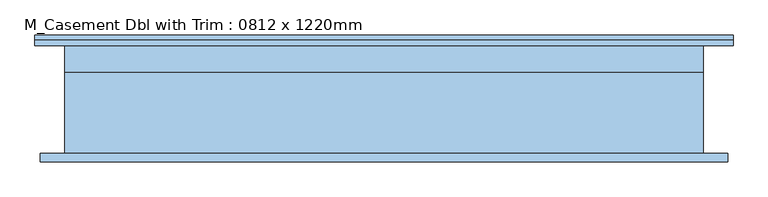
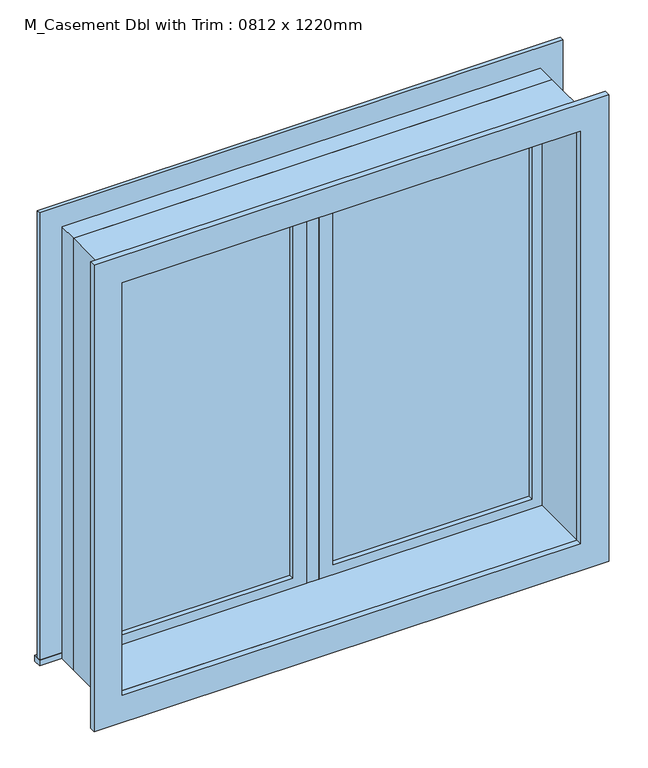
"""IFC4 building model written with IfcOpenShell, lengths in millimetres: window geometry, M_Casement Dbl with Trim : 0812 x 1220mm."""

from ifc_helpers import new_model, si_unit, frame, origin, place, context, project, spatial, polyline, outline, extrude, source, transform, mapped, element, save


def m_casement_dbl_with_trim_0812_x_1220mm_81b237b5(model_context):
    return source(origin(), model_context, "Body", "SweptSolid", [
        extrude(outline(polyline([(63.5, 111.175), (686.5, 111.175), (686.5, 98.475), (63.5, 98.475), (63.5, 111.175)])), frame((0.0, 0.0, 963.5), z_axis=(0.0, 0.0, 1.0), x_axis=(1.0, 0.0, 0.0)), (0.0, 0.0, 1.0), 1303.0),
        extrude(outline(polyline([(2310.95, 19.05), (919.05, 19.05), (919.05, 730.95), (2310.95, 730.95), (2310.95, 19.05)]), holes=[polyline([(2266.5, 63.5), (2266.5, 686.5), (963.5, 686.5), (963.5, 63.5), (2266.5, 63.5)])]), frame((0.0, 82.6, 0.0), z_axis=(0.0, 1.0, 0.0), x_axis=(0.0, 0.0, 1.0)), (0.0, 0.0, 1.0), 44.45),
        extrude(outline(polyline([(-819.95, 171.75), (819.95, 171.75), (819.95, 146.05), (-819.95, 146.05), (-819.95, 171.75)])), frame((0.0, 0.0, 900.0), z_axis=(0.0, 0.0, 1.0), x_axis=(1.0, 0.0, 0.0)), (0.0, 0.0, 1.0), 19.05),
        extrude(outline(polyline([(2310.95, -730.95), (2310.95, 730.95), (919.05, 730.95), (919.05, 819.95), (2399.95, 819.95), (2399.95, -819.95), (919.05, -819.95), (919.05, -730.95), (2310.95, -730.95)])), frame((0.0, 146.05, 0.0), z_axis=(0.0, 1.0, 0.0), x_axis=(0.0, 0.0, 1.0)), (0.0, 0.0, 1.0), 13.0),
        extrude(outline(polyline([(2387.25, 807.25), (2387.25, -807.25), (842.75, -807.25), (842.75, 807.25), (2387.25, 807.25)]), holes=[polyline([(2298.25, 718.25), (931.75, 718.25), (931.75, -718.25), (2298.25, -718.25), (2298.25, 718.25)])]), frame((0.0, -126.95, 0.0), z_axis=(0.0, 1.0, 0.0), x_axis=(0.0, 0.0, 1.0)), (0.0, 0.0, 1.0), 19.0),
        extrude(outline(polyline([(-63.5, 98.475), (-686.5, 98.475), (-686.5, 111.175), (-63.5, 111.175), (-63.5, 98.475)])), frame((0.0, 0.0, 963.5), z_axis=(0.0, 0.0, 1.0), x_axis=(1.0, 0.0, 0.0)), (0.0, 0.0, 1.0), 1303.0),
        extrude(outline(polyline([(2310.95, -730.95), (919.05, -730.95), (919.05, -19.05), (2310.95, -19.05), (2310.95, -730.95)]), holes=[polyline([(2266.5, -686.5), (2266.5, -63.5), (963.5, -63.5), (963.5, -686.5), (2266.5, -686.5)])]), frame((0.0, 82.6, 0.0), z_axis=(0.0, 1.0, 0.0), x_axis=(0.0, 0.0, 1.0)), (0.0, 0.0, 1.0), 44.45),
        extrude(outline(polyline([(2330.0, -750.0), (900.0, -750.0), (900.0, 750.0), (2330.0, 750.0), (2330.0, -750.0)]), holes=[polyline([(2298.25, -718.25), (2298.25, 718.25), (931.75, 718.25), (931.75, -718.25), (2298.25, -718.25)])]), frame((0.0, -107.95, 0.0), z_axis=(0.0, 1.0, 0.0), x_axis=(0.0, 0.0, 1.0)), (0.0, 0.0, 1.0), 190.55),
        extrude(outline(polyline([(2330.0, 750.0), (2330.0, -750.0), (900.0, -750.0), (900.0, 750.0), (2330.0, 750.0)]), holes=[polyline([(2310.95, 730.95), (919.05, 730.95), (919.05, -730.95), (2310.95, -730.95), (2310.95, 730.95)])]), frame((0.0, 82.6, 0.0), z_axis=(0.0, 1.0, 0.0), x_axis=(0.0, 0.0, 1.0)), (0.0, 0.0, 1.0), 63.45),
        extrude(outline(polyline([(19.05, 82.6), (-19.05, 82.6), (-19.05, 146.1), (19.05, 146.1), (19.05, 82.6)])), frame((0.0, 0.0, 919.05), z_axis=(0.0, 0.0, 1.0), x_axis=(1.0, 0.0, 0.0)), (0.0, 0.0, 1.0), 1391.9),
    ])


if __name__ == "__main__":
    model = new_model("IFC4")
    model_context = context("Model", 3, world=origin())
    ifc_project = project(units=[si_unit("LENGTHUNIT", "METRE", prefix="MILLI")], contexts=[model_context])
    site = spatial("IfcSite", under=ifc_project)
    building = spatial("IfcBuilding", under=site)
    placement = place(None, origin())
    m_casement_dbl_with_trim_0812_x_1220mm_shape = m_casement_dbl_with_trim_0812_x_1220mm_81b237b5(model_context)
    element("IfcWindow", 1, ObjectType="M_Casement Dbl with Trim : 0812 x 1220mm", at=placement, inside=building, context=model_context, shape_type="MappedRepresentation", body=[
        mapped(m_casement_dbl_with_trim_0812_x_1220mm_shape, transform((0.0, 0.0, 0.0), x_axis=(1.0, 0.0, 0.0), y_axis=(0.0, 1.0, 0.0), z_axis=(0.0, 0.0, 1.0))),
    ])
    save(model, "model.ifc")

# Revit data of these elements
# Type "M_Casement Dbl with Trim : 0812 x 1220mm"
#   Type Mark = "W1"
#   Construction Type Id = "GSP4R"
#   Analytic Construction = "1/8 in Pilkington single glazing"
#   Visual Light Transmittance = 0.9
#   Solar Heat Gain Coefficient = 0.78
#   Heat Transfer Coefficient (U) = 3.6886 W/(m²·K)
#   Height = 1430 mm
#   Default Sill Height = 900 mm
#   Trim Projection - Ext. = 13 mm
#   Trim Projection - Int. = 19 mm
#   Trim Width - Exterior = 89 mm
#   Trim Width - Interior = 89 mm
#   Width = 1500 mm
#   Window Inset = 19 mm
#   Glass Pane Material = Glass
#   Sash = wooden-3
#   Trim Exterior Material = wooden-3
#   Trim Interior Material = wooden-3
#   Wall Closure = (empty or 0)
# Element 1 (IfcWindow, "M_Casement Dbl with Trim : 0812 x 1220mm")
#   Materials on its faces: "wooden-3", "Glass"
# Materials
#   "Glass": class "Glass", colour RGB 140 218 255, transparency 0.75, Description = "Soda Lime Glass", Cost = 0
#   "wooden-3": class "Generic", colour RGB 120 120 120, transparency 0, Cost = 0
